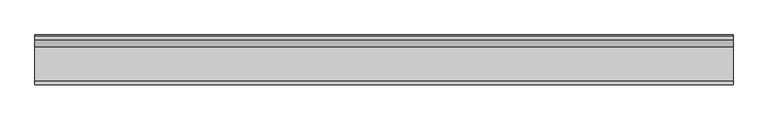
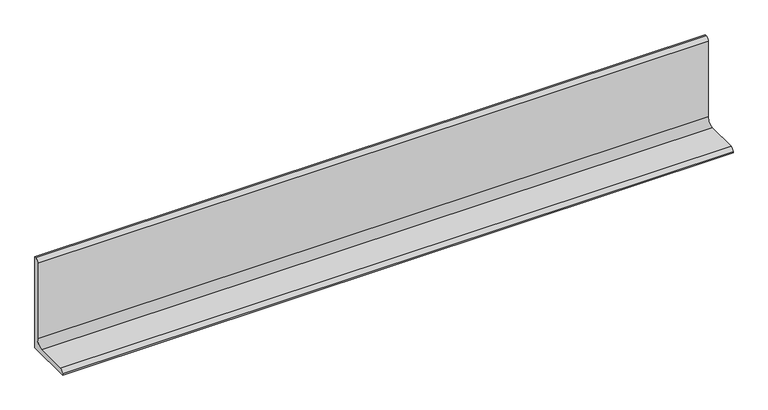
"""IFC4 building model written with IfcOpenShell, lengths in millimetres: beam geometry, NLRS_28_SF_LIB_stalen ligger hoekprofiel ongelijkzijdig-AV-MMBS-SRP_gen_rsf : stalen ligger ongelijzijdig hoekprofiel LUEQ_gen__200x100x10."""

from ifc_helpers import new_model, si_unit, point, frame, frame_2d, origin, place, context, project, spatial, polyline, circle_curve, trimmed, segment, composite_curve, outline, extrude, source, transform, mapped, element, save


def beam_132ceafd(model_context):
    return source(origin(), model_context, "Body", "SweptSolid", [
        extrude(outline(composite_curve([segment(polyline([(20.13, -69.3), (-79.87, -69.3), (-79.87, -66.8)]), True, "CONTINUOUS"), segment(trimmed(circle_curve(frame_2d((-72.37, -66.8)), 7.5), [point((-79.87, -66.8))], [point((-72.37, -59.3))], False, "CARTESIAN"), True, "CONTINUOUS"), segment(polyline([(-72.37, -59.3), (-4.87, -59.3)]), True, "CONTINUOUS"), segment(trimmed(circle_curve(frame_2d((-4.87, -44.3)), 15.0), [point((-4.87, -59.3))], [point((10.13, -44.3))], True, "CARTESIAN"), True, "CONTINUOUS"), segment(polyline([(10.13, -44.3), (10.13, 123.2)]), True, "CONTINUOUS"), segment(trimmed(circle_curve(frame_2d((17.63, 123.2)), 7.5), [point((10.13, 123.2))], [point((17.63, 130.7))], False, "CARTESIAN"), True, "CONTINUOUS"), segment(polyline([(17.63, 130.7), (20.13, 130.7), (20.13, -69.3)]), True, "CONTINUOUS")], self_intersect=False)), frame((-700.0, 0.0, 0.0), z_axis=(1.0, 0.0, 0.0), x_axis=(0.0, 1.0, 0.0)), (0.0, 0.0, 1.0), 1400.0),
    ])


if __name__ == "__main__":
    model = new_model("IFC4")
    model_context = context("Model", 3, world=origin())
    ifc_project = project(units=[si_unit("LENGTHUNIT", "METRE", prefix="MILLI")], contexts=[model_context])
    site = spatial("IfcSite", under=ifc_project)
    building = spatial("IfcBuilding", under=site)
    placement = place(None, origin())
    beam_shape = beam_132ceafd(model_context)
    element("IfcBeam", 1, ObjectType="NLRS_28_SF_LIB_stalen ligger hoekprofiel ongelijkzijdig-AV-MMBS-SRP_gen_rsf : stalen ligger ongelijzijdig hoekprofiel LUEQ_gen__200x100x10", at=placement, inside=building, context=model_context, shape_type="MappedRepresentation", body=[
        mapped(beam_shape, transform((0.0, 0.0, 0.0), x_axis=(1.0, 0.0, 0.0), y_axis=(0.0, 1.0, 0.0), z_axis=(0.0, 0.0, 1.0))),
    ])
    save(model, "model.ifc")

# Revit data of these elements
# Type "NLRS_28_SF_LIB_stalen ligger hoekprofiel ongelijkzijdig-AV-MMBS-SRP_gen_rsf : stalen ligger ongelijzijdig hoekprofiel LUEQ_gen__200x100x10"
#   Type IfcGUID = "0dxhH9VHH5jh7XQ0uLfXuR"
#   IfcExportAs = "IfcBeamType"
#   Type Comments = "L200x100x10"
#   Model = " "
#   Manufacturer = " "
#   Fire Rating = " "
#   Description = "stalen ligger L200x100x10"
#   Assembly Code = "28.11"
#   vz = 130.7 mm
#   vy = 79.87 mm
#   tw = 10 mm
#   tf = 10 mm
#   ri = 7.5 mm
#   ra = 15 mm
#   d = 200 mm
#   bf = 100 mm
#   NLRS_C_lengte [instance default] = 1524 mm
#   Length [instance default] = 1524 mm
#   Structural Material = NLRS_h2_staal_gen_rsf
#   Keynote = ""
# Element 1 (IfcBeam, "NLRS_28_SF_LIB_stalen ligger hoekprofiel ongelijkzijdig-AV-MMBS-SRP_gen_rsf : stalen ligger ongelijzijdig hoekprofiel LUEQ_gen__200x100x10")
#   NLRS_C_lengte = 1400 mm
#   Materials on its faces: "NLRS_h2_staal_gen_rsf"
# Materials
#   "NLRS_h2_staal_gen_rsf": class "H - Metaal", colour RGB 189 187 185, transparency 0, Keynote = "h2", Manufacturer = "Revit Standards Foundation", URL = "www.revitstandards.org", Description = "staal", Cost = 0
